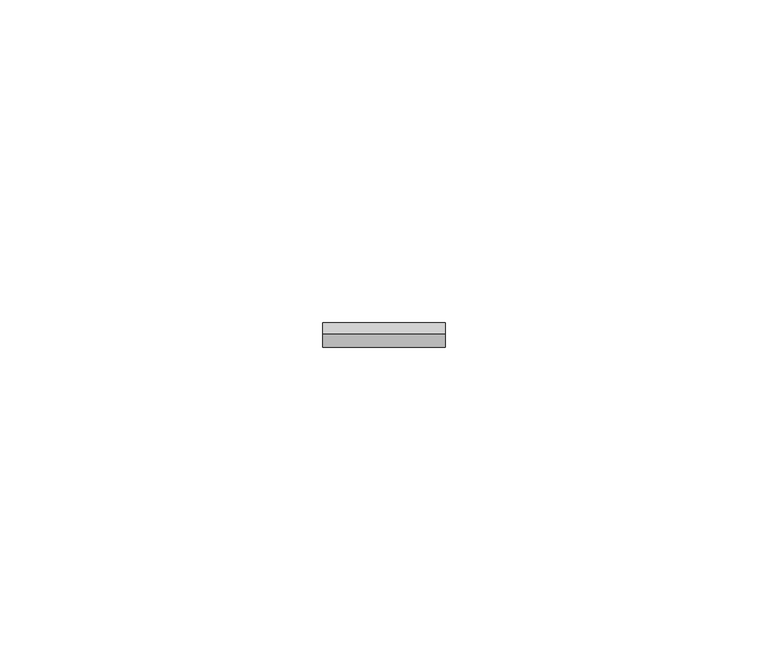
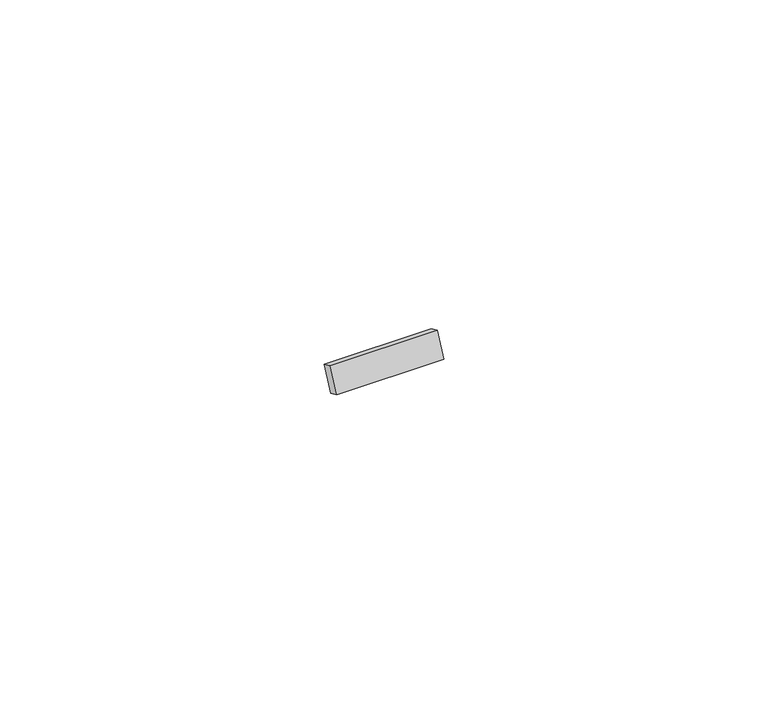
"""IFC4 building model written with IfcOpenShell, lengths in millimetres: furniture geometry, MOLDURA TELA1 : MOLDURA TELA."""

import ifcopenshell
import ifcopenshell.guid

model = None  # the IFC model being written
_history = None  # IfcOwnerHistory: only IFC2X3 demands one
_inside = {}  # id of a spatial element -> (the spatial element, [elements in it])
_under = {}  # id of a project, library or spatial element -> (it, [spatial elements below it])
_declared = {}  # id of a project -> (the project, [libraries it declares])
_typed = {}  # id of a type object -> (the type object, [elements of that type])
_made_of = {}  # id of a material, layer set ... -> (it, [elements and type objects made of it])


def new_model(schema):
    """Start an empty IFC model of exactly this schema.

    Asked for "IFC4X3", IfcOpenShell would pick the latest addendum, in which some entities
    have other attributes; the version numbers below select the first issue.
    IFC2X3 requires an IfcOwnerHistory on every rooted entity: one is made here for all.
    """
    global model, _history
    if schema == "IFC4X3":
        model = ifcopenshell.file(schema_version=(4, 3, 0, 0))
    else:
        model = ifcopenshell.file(schema=schema)
    _inside.clear()
    _under.clear()
    _declared.clear()
    _typed.clear()
    _made_of.clear()
    _history = None
    if model.schema == "IFC2X3":
        org = make("IfcOrganization", Name="unknown")
        user = make(
            "IfcPersonAndOrganization",
            ThePerson=make("IfcPerson", FamilyName="unknown"),
            TheOrganization=org,
        )
        app = make(
            "IfcApplication",
            ApplicationDeveloper=org,
            Version="unknown",
            ApplicationFullName="unknown",
            ApplicationIdentifier="unknown",
        )
        _history = make(
            "IfcOwnerHistory",
            OwningUser=user,
            OwningApplication=app,
            ChangeAction="ADDED",
            CreationDate=0,
        )
    return model


def make(cls, **values):
    """One entity of the class cls with the attributes given. An attribute that is None is left unset."""
    return model.create_entity(
        cls, **{name: value for name, value in values.items() if value is not None}
    )


def rooted(cls, **values):
    """An entity with a GlobalId (a new one), such as an element, a storey or a relation."""
    return make(cls, GlobalId=ifcopenshell.guid.new(), OwnerHistory=_history, **values)


def si_unit(unit_type, name, prefix=None):
    """IfcSIUnit, for example si_unit("LENGTHUNIT", "METRE", prefix="MILLI")."""
    return make("IfcSIUnit", UnitType=unit_type, Prefix=prefix, Name=name)


def assignment(units):
    """IfcUnitAssignment: the units of a project."""
    return None if units is None else make("IfcUnitAssignment", Units=units)


def point(xyz):
    """IfcCartesianPoint."""
    return None if xyz is None else make("IfcCartesianPoint", Coordinates=xyz)


def direction(xyz):
    """IfcDirection."""
    return None if xyz is None else make("IfcDirection", DirectionRatios=xyz)


def frame(location, z_axis=None, x_axis=None):
    """IfcAxis2Placement3D, a coordinate frame: its origin and axes. An axis left out is left unset."""
    return make(
        "IfcAxis2Placement3D",
        Location=point(location),
        Axis=direction(z_axis),
        RefDirection=direction(x_axis),
    )


def origin():
    """The frame at (0, 0, 0) with its axes left unset."""
    return frame((0.0, 0.0, 0.0))


def place(relative_to, where):
    """IfcLocalPlacement: puts the frame where relative to a parent placement (None: the world)."""
    return make(
        "IfcLocalPlacement", PlacementRelTo=relative_to, RelativePlacement=where
    )


def context(
    kind, dimensions, precision=None, world=None, true_north=None, identifier=None
):
    """IfcGeometricRepresentationContext, for example the 3D "Model" context."""
    return make(
        "IfcGeometricRepresentationContext",
        ContextIdentifier=identifier,
        ContextType=kind,
        CoordinateSpaceDimension=dimensions,
        Precision=precision,
        WorldCoordinateSystem=world,
        TrueNorth=true_north,
    )


def project(units=None, contexts=None):
    """IfcProject with its units and contexts."""
    return rooted(
        "IfcProject",
        Name="project",
        RepresentationContexts=contexts,
        UnitsInContext=assignment(units),
    )


def spatial(cls, under=None, at=None, **own):
    """A site, building, storey or space (cls), placed at a placement, below another one or the project."""
    s = rooted(cls, ObjectPlacement=at, **own)
    if under is not None:
        _under.setdefault(under.id(), (under, []))[1].append(s)
    return s


def polyline(points):
    """IfcPolyline through the points."""
    return make("IfcPolyline", Points=[point(p) for p in points])


def outline(outer, holes=None, kind="AREA"):
    """IfcArbitraryClosedProfileDef: a profile drawn as a closed curve; with holes, ...WithVoids."""
    if holes is None:
        return make("IfcArbitraryClosedProfileDef", ProfileType=kind, OuterCurve=outer)
    return make(
        "IfcArbitraryProfileDefWithVoids",
        ProfileType=kind,
        OuterCurve=outer,
        InnerCurves=holes,
    )


def extrude(swept, where, along, depth):
    """IfcExtrudedAreaSolid: the profile swept, set in the frame where, extruded along a direction by depth."""
    return make(
        "IfcExtrudedAreaSolid",
        SweptArea=swept,
        Position=where,
        ExtrudedDirection=direction(along),
        Depth=depth,
    )


def shape(context_of_items, identifier, shape_type, items):
    """IfcShapeRepresentation: the items that make up one representation, for example the "Body"."""
    return make(
        "IfcShapeRepresentation",
        ContextOfItems=context_of_items,
        RepresentationIdentifier=identifier,
        RepresentationType=shape_type,
        Items=items,
    )


def source(mapping_origin, context_of_items, identifier, shape_type, items):
    """IfcRepresentationMap: a shape defined once, which mapped items show again and again."""
    return make(
        "IfcRepresentationMap",
        MappingOrigin=mapping_origin,
        MappedRepresentation=shape(context_of_items, identifier, shape_type, items),
    )


def transform(
    local_origin,
    x_axis=None,
    y_axis=None,
    z_axis=None,
    scale=None,
    scale2=None,
    scale3=None,
    uniform=True,
):
    """IfcCartesianTransformationOperator3D, or its non-uniform kind. x_axis, y_axis, z_axis: its Axis1, 2, 3."""
    if uniform:
        return make(
            "IfcCartesianTransformationOperator3D",
            Axis1=direction(x_axis),
            Axis2=direction(y_axis),
            LocalOrigin=point(local_origin),
            Scale=scale,
            Axis3=direction(z_axis),
        )
    return make(
        "IfcCartesianTransformationOperator3DnonUniform",
        Axis1=direction(x_axis),
        Axis2=direction(y_axis),
        LocalOrigin=point(local_origin),
        Scale=scale,
        Axis3=direction(z_axis),
        Scale2=scale2,
        Scale3=scale3,
    )


def mapped(mapping_source, mapping_target):
    """IfcMappedItem: shows the shape of a source again, moved by a transform."""
    return make(
        "IfcMappedItem", MappingSource=mapping_source, MappingTarget=mapping_target
    )


def made_of(thing, what):
    """Note that an element or type object is made of a material, layer set ...; save() writes the relation."""
    if what is not None:
        _made_of.setdefault(what.id(), (what, []))[1].append(thing)
    return thing


def element(
    cls,
    number,
    at=None,
    inside=None,
    cuts=None,
    type_object=None,
    material=None,
    context=None,
    identifier="Body",
    shape_type=None,
    held_by="IfcProductDefinitionShape",
    body=None,
    shapes=None,
    **own,
):
    """One element of the class cls, such as IfcWall. Its Tag is "e" and its number.

    at: its placement. inside: the storey or other place that contains it. cuts: it is an
    opening in that element (IfcRelVoidsElement). A single representation is given by context,
    identifier, shape_type and body (its items); several are given by shapes. held_by: the class
    of the entity that holds the representations. save() writes the other relations.
    """
    e = rooted(cls, Tag="e%d" % number, ObjectPlacement=at, **own)
    if body is not None:
        shapes = [shape(context, identifier, shape_type, body)]
    if shapes is not None:
        e.Representation = make(held_by, Representations=shapes)
    if inside is not None:
        _inside.setdefault(inside.id(), (inside, []))[1].append(e)
    if cuts is not None:
        rooted(
            "IfcRelVoidsElement", RelatingBuildingElement=cuts, RelatedOpeningElement=e
        )
    if type_object is not None:
        _typed.setdefault(type_object.id(), (type_object, []))[1].append(e)
    return made_of(e, material)


def aggregate(whole, parts):
    """IfcRelAggregates: a whole, such as a stair, and the parts it consists of."""
    return rooted("IfcRelAggregates", RelatingObject=whole, RelatedObjects=parts)


def save(model, path):
    """Write the relations noted so far, then the file.

    IfcRelAggregates (storeys below a building ...), IfcRelContainedInSpatialStructure (elements
    in a storey), IfcRelDefinesByType, IfcRelAssociatesMaterial and IfcRelDeclares: one each for
    every whole, place, type object, material and project.
    """
    for whole, parts in _under.values():
        aggregate(whole, parts)
    for where, things in _inside.values():
        rooted(
            "IfcRelContainedInSpatialStructure",
            RelatedElements=things,
            RelatingStructure=where,
        )
    for kind, things in _typed.values():
        rooted("IfcRelDefinesByType", RelatedObjects=things, RelatingType=kind)
    for what, things in _made_of.values():
        rooted("IfcRelAssociatesMaterial", RelatedObjects=things, RelatingMaterial=what)
    for by, libraries in _declared.values():
        rooted("IfcRelDeclares", RelatingContext=by, RelatedDefinitions=libraries)
    model.write(path)


def furniture_bc1ec6cb(model_context):
    return source(origin(), model_context, "Body", "SweptSolid", [
        extrude(outline(polyline([(0.0, -19.0), (0.0, 0.0), (2.0, 0.0), (2.0, -19.0), (0.0, -19.0)])), frame((2400.0719295, 1317.2941444, 58.8666666), z_axis=(0.0, 0.4226182617406868, 0.9063077870366559), x_axis=(0.0, -0.9063077870366559, 0.4226182617406868)), (0.0, 0.0, 1.0), 4.7),
    ])


if __name__ == "__main__":
    model = new_model("IFC4")
    model_context = context("Model", 3, world=origin())
    ifc_project = project(units=[si_unit("LENGTHUNIT", "METRE", prefix="MILLI")], contexts=[model_context])
    site = spatial("IfcSite", under=ifc_project)
    building = spatial("IfcBuilding", under=site)
    placement = place(None, origin())
    furniture_shape = furniture_bc1ec6cb(model_context)
    element("IfcFurniture", 1, ObjectType="MOLDURA TELA1 : MOLDURA TELA", at=placement, inside=building, context=model_context, shape_type="MappedRepresentation", body=[
        mapped(furniture_shape, transform((0.0, 0.0, 0.0), x_axis=(1.0, 0.0, 0.0), y_axis=(0.0, 1.0, 0.0), z_axis=(0.0, 0.0, 1.0))),
    ])
    save(model, "model.ifc")

# Revit data of these elements
# Type "MOLDURA TELA1 : MOLDURA TELA"
#   Height = 0
# Element 1 (IfcFurniture, "MOLDURA TELA1 : MOLDURA TELA")
#   Materials on its faces: ".BOX FUNDO"
# Materials
#   ".BOX FUNDO": class "Vidro", colour RGB 236 240 239, transparency 0.15, Cost = 0
